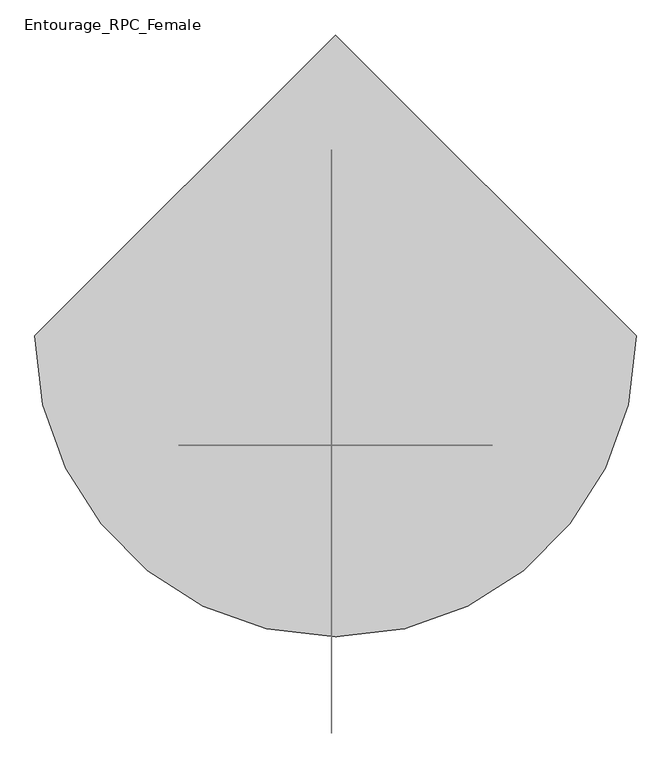
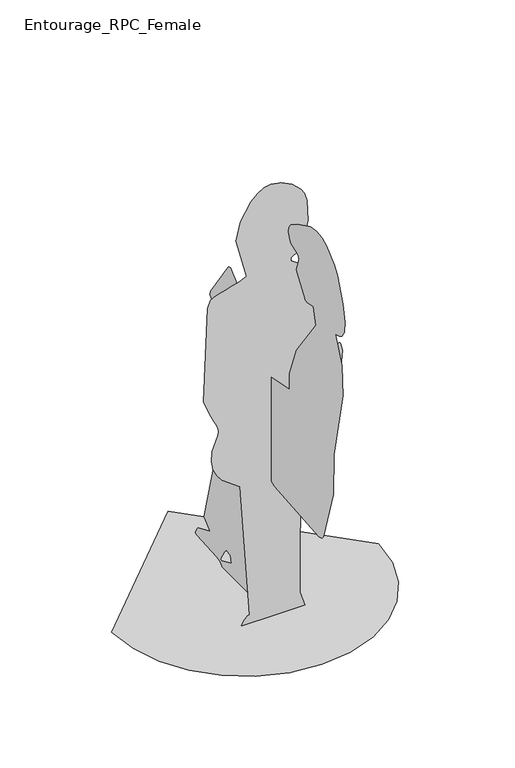
"""IFC4 building model written with IfcOpenShell, lengths in millimetres: proxy geometry, Entourage_RPC_Female : Cynthia."""

import ifcopenshell
import ifcopenshell.guid

model = None  # the IFC model being written
_history = None  # IfcOwnerHistory: only IFC2X3 demands one
_inside = {}  # id of a spatial element -> (the spatial element, [elements in it])
_under = {}  # id of a project, library or spatial element -> (it, [spatial elements below it])
_declared = {}  # id of a project -> (the project, [libraries it declares])
_typed = {}  # id of a type object -> (the type object, [elements of that type])
_made_of = {}  # id of a material, layer set ... -> (it, [elements and type objects made of it])


def new_model(schema):
    """Start an empty IFC model of exactly this schema.

    Asked for "IFC4X3", IfcOpenShell would pick the latest addendum, in which some entities
    have other attributes; the version numbers below select the first issue.
    IFC2X3 requires an IfcOwnerHistory on every rooted entity: one is made here for all.
    """
    global model, _history
    if schema == "IFC4X3":
        model = ifcopenshell.file(schema_version=(4, 3, 0, 0))
    else:
        model = ifcopenshell.file(schema=schema)
    _inside.clear()
    _under.clear()
    _declared.clear()
    _typed.clear()
    _made_of.clear()
    _history = None
    if model.schema == "IFC2X3":
        org = make("IfcOrganization", Name="unknown")
        user = make(
            "IfcPersonAndOrganization",
            ThePerson=make("IfcPerson", FamilyName="unknown"),
            TheOrganization=org,
        )
        app = make(
            "IfcApplication",
            ApplicationDeveloper=org,
            Version="unknown",
            ApplicationFullName="unknown",
            ApplicationIdentifier="unknown",
        )
        _history = make(
            "IfcOwnerHistory",
            OwningUser=user,
            OwningApplication=app,
            ChangeAction="ADDED",
            CreationDate=0,
        )
    return model


def make(cls, **values):
    """One entity of the class cls with the attributes given. An attribute that is None is left unset."""
    return model.create_entity(
        cls, **{name: value for name, value in values.items() if value is not None}
    )


def rooted(cls, **values):
    """An entity with a GlobalId (a new one), such as an element, a storey or a relation."""
    return make(cls, GlobalId=ifcopenshell.guid.new(), OwnerHistory=_history, **values)


def si_unit(unit_type, name, prefix=None):
    """IfcSIUnit, for example si_unit("LENGTHUNIT", "METRE", prefix="MILLI")."""
    return make("IfcSIUnit", UnitType=unit_type, Prefix=prefix, Name=name)


def assignment(units):
    """IfcUnitAssignment: the units of a project."""
    return None if units is None else make("IfcUnitAssignment", Units=units)


def point(xyz):
    """IfcCartesianPoint."""
    return None if xyz is None else make("IfcCartesianPoint", Coordinates=xyz)


def direction(xyz):
    """IfcDirection."""
    return None if xyz is None else make("IfcDirection", DirectionRatios=xyz)


def frame(location, z_axis=None, x_axis=None):
    """IfcAxis2Placement3D, a coordinate frame: its origin and axes. An axis left out is left unset."""
    return make(
        "IfcAxis2Placement3D",
        Location=point(location),
        Axis=direction(z_axis),
        RefDirection=direction(x_axis),
    )


def origin():
    """The frame at (0, 0, 0) with its axes left unset."""
    return frame((0.0, 0.0, 0.0))


def place(relative_to, where):
    """IfcLocalPlacement: puts the frame where relative to a parent placement (None: the world)."""
    return make(
        "IfcLocalPlacement", PlacementRelTo=relative_to, RelativePlacement=where
    )


def context(
    kind, dimensions, precision=None, world=None, true_north=None, identifier=None
):
    """IfcGeometricRepresentationContext, for example the 3D "Model" context."""
    return make(
        "IfcGeometricRepresentationContext",
        ContextIdentifier=identifier,
        ContextType=kind,
        CoordinateSpaceDimension=dimensions,
        Precision=precision,
        WorldCoordinateSystem=world,
        TrueNorth=true_north,
    )


def project(units=None, contexts=None):
    """IfcProject with its units and contexts."""
    return rooted(
        "IfcProject",
        Name="project",
        RepresentationContexts=contexts,
        UnitsInContext=assignment(units),
    )


def spatial(cls, under=None, at=None, **own):
    """A site, building, storey or space (cls), placed at a placement, below another one or the project."""
    s = rooted(cls, ObjectPlacement=at, **own)
    if under is not None:
        _under.setdefault(under.id(), (under, []))[1].append(s)
    return s


def point_list(points):
    """IfcCartesianPointList2D or 3D."""
    cls = (
        "IfcCartesianPointList2D" if len(points[0]) == 2 else "IfcCartesianPointList3D"
    )
    return make(cls, CoordList=points)


def triangles(points, corners, closed=None, point_numbers=None):
    """IfcTriangulatedFaceSet: each triangle names its three corners, points numbered from 1."""
    return make(
        "IfcTriangulatedFaceSet",
        Coordinates=point_list(points),
        Closed=closed,
        CoordIndex=corners,
        PnIndex=point_numbers,
    )


def shape(context_of_items, identifier, shape_type, items):
    """IfcShapeRepresentation: the items that make up one representation, for example the "Body"."""
    return make(
        "IfcShapeRepresentation",
        ContextOfItems=context_of_items,
        RepresentationIdentifier=identifier,
        RepresentationType=shape_type,
        Items=items,
    )


def source(mapping_origin, context_of_items, identifier, shape_type, items):
    """IfcRepresentationMap: a shape defined once, which mapped items show again and again."""
    return make(
        "IfcRepresentationMap",
        MappingOrigin=mapping_origin,
        MappedRepresentation=shape(context_of_items, identifier, shape_type, items),
    )


def transform(
    local_origin,
    x_axis=None,
    y_axis=None,
    z_axis=None,
    scale=None,
    scale2=None,
    scale3=None,
    uniform=True,
):
    """IfcCartesianTransformationOperator3D, or its non-uniform kind. x_axis, y_axis, z_axis: its Axis1, 2, 3."""
    if uniform:
        return make(
            "IfcCartesianTransformationOperator3D",
            Axis1=direction(x_axis),
            Axis2=direction(y_axis),
            LocalOrigin=point(local_origin),
            Scale=scale,
            Axis3=direction(z_axis),
        )
    return make(
        "IfcCartesianTransformationOperator3DnonUniform",
        Axis1=direction(x_axis),
        Axis2=direction(y_axis),
        LocalOrigin=point(local_origin),
        Scale=scale,
        Axis3=direction(z_axis),
        Scale2=scale2,
        Scale3=scale3,
    )


def mapped(mapping_source, mapping_target):
    """IfcMappedItem: shows the shape of a source again, moved by a transform."""
    return make(
        "IfcMappedItem", MappingSource=mapping_source, MappingTarget=mapping_target
    )


def made_of(thing, what):
    """Note that an element or type object is made of a material, layer set ...; save() writes the relation."""
    if what is not None:
        _made_of.setdefault(what.id(), (what, []))[1].append(thing)
    return thing


def element(
    cls,
    number,
    at=None,
    inside=None,
    cuts=None,
    type_object=None,
    material=None,
    context=None,
    identifier="Body",
    shape_type=None,
    held_by="IfcProductDefinitionShape",
    body=None,
    shapes=None,
    **own,
):
    """One element of the class cls, such as IfcWall. Its Tag is "e" and its number.

    at: its placement. inside: the storey or other place that contains it. cuts: it is an
    opening in that element (IfcRelVoidsElement). A single representation is given by context,
    identifier, shape_type and body (its items); several are given by shapes. held_by: the class
    of the entity that holds the representations. save() writes the other relations.
    """
    e = rooted(cls, Tag="e%d" % number, ObjectPlacement=at, **own)
    if body is not None:
        shapes = [shape(context, identifier, shape_type, body)]
    if shapes is not None:
        e.Representation = make(held_by, Representations=shapes)
    if inside is not None:
        _inside.setdefault(inside.id(), (inside, []))[1].append(e)
    if cuts is not None:
        rooted(
            "IfcRelVoidsElement", RelatingBuildingElement=cuts, RelatedOpeningElement=e
        )
    if type_object is not None:
        _typed.setdefault(type_object.id(), (type_object, []))[1].append(e)
    return made_of(e, material)


def aggregate(whole, parts):
    """IfcRelAggregates: a whole, such as a stair, and the parts it consists of."""
    return rooted("IfcRelAggregates", RelatingObject=whole, RelatedObjects=parts)


def save(model, path):
    """Write the relations noted so far, then the file.

    IfcRelAggregates (storeys below a building ...), IfcRelContainedInSpatialStructure (elements
    in a storey), IfcRelDefinesByType, IfcRelAssociatesMaterial and IfcRelDeclares: one each for
    every whole, place, type object, material and project.
    """
    for whole, parts in _under.values():
        aggregate(whole, parts)
    for where, things in _inside.values():
        rooted(
            "IfcRelContainedInSpatialStructure",
            RelatedElements=things,
            RelatingStructure=where,
        )
    for kind, things in _typed.values():
        rooted("IfcRelDefinesByType", RelatedObjects=things, RelatingType=kind)
    for what, things in _made_of.values():
        rooted("IfcRelAssociatesMaterial", RelatedObjects=things, RelatingMaterial=what)
    for by, libraries in _declared.values():
        rooted("IfcRelDeclares", RelatingContext=by, RelatedDefinitions=libraries)
    model.write(path)


def entourage_rpc_female_c3b5a3e1(model_context):
    return source(origin(), model_context, "Body", "Tessellation", [
        triangles([(-437.3060472, 0.0, 2.93e-05), (-425.7451249, -100.2016327, 2.93e-05), (-392.8196637, -192.220807, 2.93e-05), (-341.1660942, -273.421065, 2.93e-05), (-273.4210832, -341.1661669, 2.93e-05), (-192.2207525, -392.8196274, 2.93e-05), (-100.2015873, -425.7450522, 2.93e-05), (1.91e-05, -437.3060472, 2.93e-05), (100.2016418, -425.7451249, 2.93e-05), (192.2208252, -392.8196637, 2.93e-05), (273.4210832, -341.1660942, 2.93e-05), (341.1662395, -273.4210832, 2.93e-05), (392.8196274, -192.2207344, 2.93e-05), (425.7450522, -100.2015691, 2.93e-05), (437.3060472, 3.36e-05, 2.93e-05), (-5.73e-05, 437.3060835, 2.93e-05), (-5.5814595, 72.2469164, 69.4963894), (-5.5814595, 67.0311828, 46.0256926), (-5.5814618, 124.4040072, 19.9471473), (-5.5814618, 129.6197135, 25.1628355), (-5.5814606, 107.6002908, 62.2269748), (-5.5814595, 95.7176132, 74.7120821), (-5.5814595, -28.6037251, 4.4e-06), (-5.5814589, -39.8908927, 35.5942709), (-5.5814589, -42.4985824, 37.2668455), (-5.5814583, -45.6386024, 39.1828236), (-5.5814583, -48.9915681, 41.1595925), (-5.5814583, -52.2381586, 43.0148617), (-5.5814583, -55.0589485, 44.5657618), (-5.5814583, -57.1346439, 45.630268), (-5.5814583, -58.1458422, 46.0256972), (-5.5814595, -58.1459239, 5.3e-06), (-5.5814589, -108.9534877, 6.8e-06), (-5.5814578, -116.5758876, 29.8220396), (-5.5814544, -109.3237594, 163.617066), (-5.5814447, -45.4571863, 488.7460396), (-5.5814447, -47.7144613, 510.22398), (-5.5814447, -52.930154, 512.8317787), (-5.5814442, -176.693648, 461.1355883), (-5.5814407, -431.0103195, 441.4519423), (-5.5814407, -446.7163739, 445.0275962), (-5.5814402, -456.1588572, 455.8254473), (-5.5814334, -511.6812675, 636.0533998), (-5.5814294, -514.5206291, 776.2252218), (-5.581422, -566.7675127, 1012.4535353), (-5.5814192, -561.4620226, 1112.6385538), (-5.5814163, -522.3441341, 1198.6978357), (-5.5814163, -544.766203, 1204.597403), (-5.5814158, -561.2101121, 1214.9823069), (-5.5814152, -573.9146782, 1236.2579704), (-5.5814135, -577.4590839, 1272.8749214), (-5.5814124, -566.4222939, 1329.2833969), (-5.5814107, -535.3834182, 1409.9341427), (-5.5814101, -516.7875329, 1433.7646648), (-5.5814095, -472.5757693, 1474.3213463), (-5.5814095, -445.9834971, 1486.7823589), (-5.5814101, -415.7492961, 1491.1889214), (-5.5814107, -381.3848602, 1485.4078789), (-5.5814124, -308.1104447, 1450.1712215), (-5.5814135, -271.6909563, 1426.3745636), (-5.5814141, -259.9824413, 1410.5522736), (-5.5814152, -256.5010404, 1391.3537361), (-5.5814158, -264.1664701, 1368.2083466), (-5.5814158, -270.5527808, 1361.5173306), (-5.5814158, -307.4895524, 1345.9739479), (-5.5814158, -313.689719, 1341.0972107), (-5.5814158, -316.3235335, 1334.3062008), (-5.5814163, -314.5106718, 1321.5905525), (-5.5814175, -303.2843222, 1289.972715), (-5.5814175, -303.9330653, 1281.3193188), (-5.5814186, -344.8554039, 1227.4574902), (-5.5814192, -350.225752, 1216.9527534), (-5.5814192, -354.0102593, 1213.1380154), (-5.5814192, -360.9106739, 1211.8318451), (-5.581418, -397.1671454, 1216.9527534), (-5.5814197, -412.8142282, 1162.1877823), (-5.5814254, -300.7219422, 1007.465613), (-5.5814294, -262.9223781, 903.7025425), (-5.5814311, -261.5586532, 849.245256), (-5.5814334, -151.2455011, 828.1027239), (-5.5814334, -131.1658673, 828.382358), (-5.5814322, -146.9134072, 873.4852736), (-5.5814322, -146.8129955, 875.3236788), (-5.5814322, -136.528476, 880.5995195), (-5.5814294, 66.2908937, 1062.7625284), (-5.5814294, 72.9542315, 1068.1179428), (-5.58143, 85.3176393, 1063.7725685), (-5.5814356, 186.9121194, 916.7362673), (-5.5814362, 189.6004001, 904.0100819), (-5.5814373, 74.8547605, 802.3037899), (-5.5814385, 53.5232047, 768.5295433), (-5.5814385, 40.9526375, 757.9702314), (-5.5814385, 7.0502453, 750.1467264), (-5.5814396, -30.7395867, 681.3431499), (-5.5814396, -32.0672991, 677.1266922), (-5.5814402, -2.7970188, 673.1422697), (-5.5814413, 74.8547605, 666.6952068), (-5.5814606, 223.5024732, 113.8299342), (-5.5814606, 192.3028696, 86.4272827), (-5.5814606, 189.6004001, 82.5356507), (-5.5814629, 257.4046916, 53.8492703), (-5.5814629, 261.0574302, 50.6335736), (-5.5814635, 266.9933869, 41.9573681), (-5.5814635, 270.402463, 33.1798516), (-5.5814635, 270.8967278, 29.8373366), (-5.5814635, 270.4438667, 27.7706795), (-5.5814635, 262.2121017, 24.672413), (-5.5814623, 148.399036, 17.7234889), (-5.5814623, 129.6197135, 12.1235673), (-5.5814623, 119.228015, 0.0), (-103.2161744, -158.8626324, 3.1383159), (-93.5649829, -158.8626324, 19.2429933), (-88.6212531, -158.8626324, 24.4594445), (-82.9718341, -158.8626324, 28.4095327), (-76.7114059, -158.8626324, 30.3785123), (-108.0056803, -158.8626688, 484.1452303), (-166.5179246, -158.8626688, 527.9972775), (-183.6323596, -158.8626688, 549.7335234), (-196.1560501, -158.8626688, 575.2326937), (-202.051348, -158.8626688, 604.6170193), (-199.2806414, -158.8626688, 638.0087311), (-180.7338447, -158.8626688, 688.9253906), (-179.5105545, -158.8626688, 700.1741953), (-181.0256691, -158.8626688, 711.0286926), (-186.0299967, -158.8626688, 724.8032879), (-192.7432497, -158.8626688, 739.7140783), (-208.556347, -158.8626688, 771.7153954), (-227.9670263, -158.8626688, 820.5585623), (-215.5927998, -158.8627051, 1139.719677), (-204.4963295, -158.8627051, 1164.795472), (-195.7042972, -158.8627051, 1170.2251551), (-178.3999392, -158.8627051, 1176.5906822), (-156.0961225, -158.8627051, 1183.4371393), (-132.3056233, -158.8627051, 1190.3085222), (-110.5413813, -158.8627051, 1196.7500622), (-94.3161544, -158.8627051, 1202.3061911), (-87.1428368, -158.8627051, 1206.5211954), (-121.0449553, -158.8627051, 1339.5217255), (-105.9598841, -158.8627233, 1402.4776211), (-72.2006802, -158.8627233, 1459.3937691), (-51.1399244, -158.8627233, 1480.6096252), (-28.7965753, -158.8627233, 1494.3423626), (-6.2993163, -158.8627233, 1498.6009689), (28.3786116, -158.8627233, 1491.3014145), (62.9444138, -158.8627233, 1473.3404469), (92.2084978, -158.8627233, 1445.5319698), (103.2306357, -158.8627233, 1428.1888424), (112.1217082, -158.8627233, 1400.9906479), (114.2135863, -158.8627051, 1329.2272957), (96.1615087, -158.8627051, 1258.9099308), (79.8726138, -158.8627051, 1233.5191841), (58.8970909, -158.8627051, 1219.5604431), (58.8970909, -158.8627051, 1209.1289577), (105.4403209, -158.8627051, 1177.1577988), (186.6819918, -158.8627051, 1146.5404089), (190.9102947, -158.8627051, 1130.2535397), (197.4606216, -158.8627051, 874.561952), (217.1153449, -158.8627051, 870.6129925), (219.4355885, -158.8627051, 869.5271576), (221.3550207, -158.8627051, 866.9867603), (227.9670444, -158.8626688, 839.7671282), (217.976248, -158.8626688, 726.675848), (216.7788284, -158.8626688, 725.5374001), (198.4189752, -158.8626688, 721.3537165), (197.1134226, -158.8626688, 721.4601053), (188.2935758, -158.8626688, 736.0854481), (176.2505791, -158.8626688, 750.1465811), (172.5435924, -158.8626688, 744.3788372), (169.4577161, -158.8626688, 737.624235), (166.7655839, -158.8626688, 730.2871828), (164.2398296, -158.8626688, 722.7722345), (161.6531779, -158.8626688, 715.4839439), (158.7782626, -158.8626688, 708.8267195), (155.3877173, -158.8626688, 703.2051149), (164.598892, -158.8626688, 582.3868355), (159.7289131, -158.8626688, 557.9940293), (150.1720292, -158.8626688, 536.3024028), (143.4522449, -158.8626688, 528.6089407), (105.4337806, -158.8626688, 509.5450607), (96.8766176, -158.8626688, 503.2558007), (90.1913244, -158.8626688, 494.5766793), (88.7456459, -158.8626324, 49.410397), (105.4366693, -158.8626324, 7.4e-05), (-104.3910663, -158.8626324, 7.4e-05)], [[15, 16, 1], [14, 15, 1], [14, 1, 2], [13, 14, 2], [13, 2, 3], [13, 3, 4], [12, 13, 4], [11, 12, 4], [11, 4, 5], [11, 5, 6], [11, 6, 7], [11, 7, 8], [11, 8, 9], [11, 9, 10], [23, 17, 18], [110, 23, 18], [110, 18, 19], [109, 110, 19], [17, 23, 24], [31, 32, 33], [31, 33, 34], [109, 19, 20], [108, 109, 20], [88, 89, 90], [82, 83, 84], [85, 86, 87], [105, 106, 107], [104, 105, 107], [103, 104, 107], [102, 103, 107], [101, 102, 107], [100, 101, 107], [100, 107, 108], [100, 108, 20], [100, 20, 21], [100, 21, 22], [87, 88, 90], [85, 87, 90], [84, 85, 90], [84, 90, 91], [84, 91, 92], [84, 92, 93], [82, 84, 93], [81, 82, 93], [81, 93, 94], [80, 81, 94], [80, 94, 95], [99, 100, 22], [17, 24, 25], [17, 25, 26], [31, 34, 35], [30, 31, 35], [17, 26, 27], [17, 27, 28], [17, 28, 29], [29, 30, 35], [17, 29, 35], [22, 17, 35], [99, 22, 35], [98, 99, 35], [97, 98, 35], [97, 35, 36], [97, 36, 37], [96, 97, 37], [96, 37, 38], [95, 96, 38], [80, 95, 38], [80, 38, 39], [79, 80, 39], [79, 39, 40], [79, 40, 41], [79, 41, 42], [79, 42, 43], [79, 43, 44], [78, 79, 44], [77, 78, 44], [77, 44, 45], [77, 45, 46], [76, 77, 46], [76, 46, 47], [75, 76, 47], [72, 73, 74], [71, 72, 74], [61, 62, 63], [60, 61, 63], [60, 63, 64], [59, 60, 64], [59, 64, 65], [59, 65, 66], [58, 59, 66], [57, 58, 66], [56, 57, 66], [55, 56, 66], [54, 55, 66], [54, 66, 67], [53, 54, 67], [52, 53, 67], [52, 67, 68], [51, 52, 68], [50, 51, 68], [49, 50, 68], [48, 49, 68], [47, 48, 68], [75, 47, 68], [74, 75, 68], [71, 74, 68], [70, 71, 68], [69, 70, 68], [183, 184, 111], [183, 111, 112], [183, 112, 113], [183, 113, 114], [183, 114, 115], [182, 183, 115], [181, 182, 115], [181, 115, 116], [154, 155, 156], [164, 165, 166], [180, 181, 116], [163, 164, 166], [162, 163, 166], [162, 166, 167], [161, 162, 167], [160, 161, 167], [159, 160, 167], [158, 159, 167], [157, 158, 167], [180, 116, 117], [180, 117, 118], [180, 118, 119], [180, 119, 120], [180, 120, 121], [180, 121, 122], [179, 180, 122], [179, 122, 123], [178, 179, 123], [177, 178, 123], [176, 177, 123], [175, 176, 123], [174, 175, 123], [174, 123, 124], [174, 124, 125], [173, 174, 125], [172, 173, 125], [171, 172, 125], [170, 171, 125], [169, 170, 125], [169, 125, 126], [168, 169, 126], [168, 126, 127], [167, 168, 127], [157, 167, 127], [157, 127, 128], [156, 157, 128], [154, 156, 128], [153, 154, 128], [153, 128, 129], [153, 129, 130], [153, 130, 131], [153, 131, 132], [153, 132, 133], [153, 133, 134], [153, 134, 135], [153, 135, 136], [153, 136, 137], [152, 153, 137], [151, 152, 137], [150, 151, 137], [149, 150, 137], [149, 137, 138], [149, 138, 139], [148, 149, 139], [147, 148, 139], [146, 147, 139], [146, 139, 140], [145, 146, 140], [145, 140, 141], [144, 145, 141], [144, 141, 142], [144, 142, 143]], closed=False),
    ])


if __name__ == "__main__":
    model = new_model("IFC4")
    model_context = context("Model", 3, world=origin())
    ifc_project = project(units=[si_unit("LENGTHUNIT", "METRE", prefix="MILLI")], contexts=[model_context])
    site = spatial("IfcSite", under=ifc_project)
    building = spatial("IfcBuilding", under=site)
    placement = place(None, origin())
    entourage_rpc_female_shape = entourage_rpc_female_c3b5a3e1(model_context)
    element("IfcBuildingElementProxy", 1, Name="Entourage_RPC_Female : Cynthia", ObjectType="Entourage_RPC_Female : Cynthia", at=placement, inside=building, context=model_context, shape_type="MappedRepresentation", body=[
        mapped(entourage_rpc_female_shape, transform((0.0, 0.0, 0.0), x_axis=(1.0, 0.0, 0.0), y_axis=(0.0, 1.0, 0.0), z_axis=(0.0, 0.0, 1.0))),
    ])
    save(model, "model.ifc")

# Revit data of these elements
# Type "Entourage_RPC_Female : Cynthia"
#   built-in parameter 1005198 = "{2, 15},{22, RPC-8-FXA2-QQQ0-UGV2-6},{1, 0},{1, 0},{2, 15},{1, 8},{5, Color},{1, 0},{1, 0},{3, 0.8},{3, 0.8},{3, 0.8},{1, 8},{7, BBoxMin},{1, 0},{1, 0},{1, 0},{1, 0},{1, 0},{1, 8},{7, BBoxMax},{1, 0},{1, 0},{1, 0},{1, 0},{1, 0},{2, 11},{9, RPCTypeId},{1, 0},{1, 0},{22, RPC-8-FXA2-QQQ0-UGV2-6},{1, 6},{14, RPCPlantHeight},{1, 0},{1, 0},{7, 4.91667},{2, 11},{7, keyword},{1, 0},{1, 0},{43, :RPCs:People [Seated-Business]:Geometry:RPC},{2, 11},{8, category},{1, 0},{1, 0},{24, People [Seated-Business]},{2, 11},{12, LocalizedUID},{1, 0},{1, 0},{7, Cynthia},{2, 14},{6, Height},{1, 0},{1, 0},{7, 4.91667},{1, 2},{16, Cast Reflections},{1, 0},{1, 0},{1, 0},{1, 2},{6, Jitter},{1, 0},{1, 0},{1, 1},{1, 2},{9, Billboard},{1, 0},{1, 0},{1, 0},{1, 2},{12, Cast Shadows},{1, 0},{1, 0},{1, 1},{1, 2},{20, Apply Filter Effects},{1, 0},{1, 0},{1, 0},{2, 11},{28, Apply Filter Effects-Text-FC},{1, 0},{1, 0},{4, None},{21, assetlibrary_base.fbx},{1, 5},"
#   built-in parameter 1005195 = "RPC-8-FXA2-QQQ0-UGV2-6"
#   Height = 0
